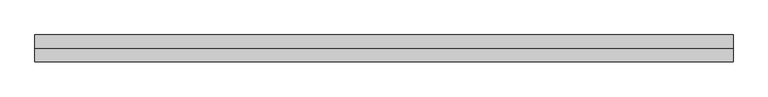
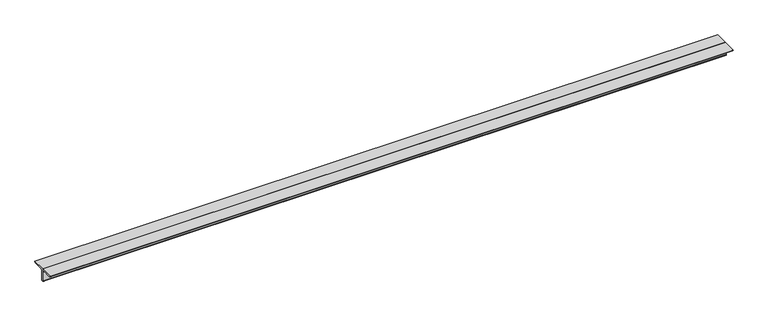
"""IFC4 building model written with IfcOpenShell, lengths in millimetres: member geometry, Steel Framing_2Ls_KS : H_SB_AR_S02_2Ls-100x100x10_VBR1."""

import ifcopenshell
import ifcopenshell.guid

model = None  # the IFC model being written
_history = None  # IfcOwnerHistory: only IFC2X3 demands one
_inside = {}  # id of a spatial element -> (the spatial element, [elements in it])
_under = {}  # id of a project, library or spatial element -> (it, [spatial elements below it])
_declared = {}  # id of a project -> (the project, [libraries it declares])
_typed = {}  # id of a type object -> (the type object, [elements of that type])
_made_of = {}  # id of a material, layer set ... -> (it, [elements and type objects made of it])


def new_model(schema):
    """Start an empty IFC model of exactly this schema.

    Asked for "IFC4X3", IfcOpenShell would pick the latest addendum, in which some entities
    have other attributes; the version numbers below select the first issue.
    IFC2X3 requires an IfcOwnerHistory on every rooted entity: one is made here for all.
    """
    global model, _history
    if schema == "IFC4X3":
        model = ifcopenshell.file(schema_version=(4, 3, 0, 0))
    else:
        model = ifcopenshell.file(schema=schema)
    _inside.clear()
    _under.clear()
    _declared.clear()
    _typed.clear()
    _made_of.clear()
    _history = None
    if model.schema == "IFC2X3":
        org = make("IfcOrganization", Name="unknown")
        user = make(
            "IfcPersonAndOrganization",
            ThePerson=make("IfcPerson", FamilyName="unknown"),
            TheOrganization=org,
        )
        app = make(
            "IfcApplication",
            ApplicationDeveloper=org,
            Version="unknown",
            ApplicationFullName="unknown",
            ApplicationIdentifier="unknown",
        )
        _history = make(
            "IfcOwnerHistory",
            OwningUser=user,
            OwningApplication=app,
            ChangeAction="ADDED",
            CreationDate=0,
        )
    return model


def make(cls, **values):
    """One entity of the class cls with the attributes given. An attribute that is None is left unset."""
    return model.create_entity(
        cls, **{name: value for name, value in values.items() if value is not None}
    )


def rooted(cls, **values):
    """An entity with a GlobalId (a new one), such as an element, a storey or a relation."""
    return make(cls, GlobalId=ifcopenshell.guid.new(), OwnerHistory=_history, **values)


def si_unit(unit_type, name, prefix=None):
    """IfcSIUnit, for example si_unit("LENGTHUNIT", "METRE", prefix="MILLI")."""
    return make("IfcSIUnit", UnitType=unit_type, Prefix=prefix, Name=name)


def assignment(units):
    """IfcUnitAssignment: the units of a project."""
    return None if units is None else make("IfcUnitAssignment", Units=units)


def point(xyz):
    """IfcCartesianPoint."""
    return None if xyz is None else make("IfcCartesianPoint", Coordinates=xyz)


def direction(xyz):
    """IfcDirection."""
    return None if xyz is None else make("IfcDirection", DirectionRatios=xyz)


def frame(location, z_axis=None, x_axis=None):
    """IfcAxis2Placement3D, a coordinate frame: its origin and axes. An axis left out is left unset."""
    return make(
        "IfcAxis2Placement3D",
        Location=point(location),
        Axis=direction(z_axis),
        RefDirection=direction(x_axis),
    )


def frame_2d(location, x_axis=None):
    """IfcAxis2Placement2D, a coordinate frame in the plane: its origin and x axis."""
    return make(
        "IfcAxis2Placement2D", Location=point(location), RefDirection=direction(x_axis)
    )


def origin():
    """The frame at (0, 0, 0) with its axes left unset."""
    return frame((0.0, 0.0, 0.0))


def place(relative_to, where):
    """IfcLocalPlacement: puts the frame where relative to a parent placement (None: the world)."""
    return make(
        "IfcLocalPlacement", PlacementRelTo=relative_to, RelativePlacement=where
    )


def context(
    kind, dimensions, precision=None, world=None, true_north=None, identifier=None
):
    """IfcGeometricRepresentationContext, for example the 3D "Model" context."""
    return make(
        "IfcGeometricRepresentationContext",
        ContextIdentifier=identifier,
        ContextType=kind,
        CoordinateSpaceDimension=dimensions,
        Precision=precision,
        WorldCoordinateSystem=world,
        TrueNorth=true_north,
    )


def project(units=None, contexts=None):
    """IfcProject with its units and contexts."""
    return rooted(
        "IfcProject",
        Name="project",
        RepresentationContexts=contexts,
        UnitsInContext=assignment(units),
    )


def spatial(cls, under=None, at=None, **own):
    """A site, building, storey or space (cls), placed at a placement, below another one or the project."""
    s = rooted(cls, ObjectPlacement=at, **own)
    if under is not None:
        _under.setdefault(under.id(), (under, []))[1].append(s)
    return s


def polyline(points):
    """IfcPolyline through the points."""
    return make("IfcPolyline", Points=[point(p) for p in points])


def circle_curve(where, radius):
    """IfcCircle in the frame where."""
    return make("IfcCircle", Position=where, Radius=radius)


def trimmed(basis, trim1, trim2, sense, master):
    """IfcTrimmedCurve: the piece of a basis curve between two trims."""
    return make(
        "IfcTrimmedCurve",
        BasisCurve=basis,
        Trim1=trim1,
        Trim2=trim2,
        SenseAgreement=sense,
        MasterRepresentation=master,
    )


def segment(curve, same_sense, transition):
    """IfcCompositeCurveSegment."""
    return make(
        "IfcCompositeCurveSegment",
        Transition=transition,
        SameSense=same_sense,
        ParentCurve=curve,
    )


def composite_curve(segments, self_intersect=None):
    """IfcCompositeCurve: segments joined end to end."""
    return make("IfcCompositeCurve", Segments=segments, SelfIntersect=self_intersect)


def outline(outer, holes=None, kind="AREA"):
    """IfcArbitraryClosedProfileDef: a profile drawn as a closed curve; with holes, ...WithVoids."""
    if holes is None:
        return make("IfcArbitraryClosedProfileDef", ProfileType=kind, OuterCurve=outer)
    return make(
        "IfcArbitraryProfileDefWithVoids",
        ProfileType=kind,
        OuterCurve=outer,
        InnerCurves=holes,
    )


def extrude(swept, where, along, depth):
    """IfcExtrudedAreaSolid: the profile swept, set in the frame where, extruded along a direction by depth."""
    return make(
        "IfcExtrudedAreaSolid",
        SweptArea=swept,
        Position=where,
        ExtrudedDirection=direction(along),
        Depth=depth,
    )


def shape(context_of_items, identifier, shape_type, items):
    """IfcShapeRepresentation: the items that make up one representation, for example the "Body"."""
    return make(
        "IfcShapeRepresentation",
        ContextOfItems=context_of_items,
        RepresentationIdentifier=identifier,
        RepresentationType=shape_type,
        Items=items,
    )


def source(mapping_origin, context_of_items, identifier, shape_type, items):
    """IfcRepresentationMap: a shape defined once, which mapped items show again and again."""
    return make(
        "IfcRepresentationMap",
        MappingOrigin=mapping_origin,
        MappedRepresentation=shape(context_of_items, identifier, shape_type, items),
    )


def transform(
    local_origin,
    x_axis=None,
    y_axis=None,
    z_axis=None,
    scale=None,
    scale2=None,
    scale3=None,
    uniform=True,
):
    """IfcCartesianTransformationOperator3D, or its non-uniform kind. x_axis, y_axis, z_axis: its Axis1, 2, 3."""
    if uniform:
        return make(
            "IfcCartesianTransformationOperator3D",
            Axis1=direction(x_axis),
            Axis2=direction(y_axis),
            LocalOrigin=point(local_origin),
            Scale=scale,
            Axis3=direction(z_axis),
        )
    return make(
        "IfcCartesianTransformationOperator3DnonUniform",
        Axis1=direction(x_axis),
        Axis2=direction(y_axis),
        LocalOrigin=point(local_origin),
        Scale=scale,
        Axis3=direction(z_axis),
        Scale2=scale2,
        Scale3=scale3,
    )


def mapped(mapping_source, mapping_target):
    """IfcMappedItem: shows the shape of a source again, moved by a transform."""
    return make(
        "IfcMappedItem", MappingSource=mapping_source, MappingTarget=mapping_target
    )


def made_of(thing, what):
    """Note that an element or type object is made of a material, layer set ...; save() writes the relation."""
    if what is not None:
        _made_of.setdefault(what.id(), (what, []))[1].append(thing)
    return thing


def element(
    cls,
    number,
    at=None,
    inside=None,
    cuts=None,
    type_object=None,
    material=None,
    context=None,
    identifier="Body",
    shape_type=None,
    held_by="IfcProductDefinitionShape",
    body=None,
    shapes=None,
    **own,
):
    """One element of the class cls, such as IfcWall. Its Tag is "e" and its number.

    at: its placement. inside: the storey or other place that contains it. cuts: it is an
    opening in that element (IfcRelVoidsElement). A single representation is given by context,
    identifier, shape_type and body (its items); several are given by shapes. held_by: the class
    of the entity that holds the representations. save() writes the other relations.
    """
    e = rooted(cls, Tag="e%d" % number, ObjectPlacement=at, **own)
    if body is not None:
        shapes = [shape(context, identifier, shape_type, body)]
    if shapes is not None:
        e.Representation = make(held_by, Representations=shapes)
    if inside is not None:
        _inside.setdefault(inside.id(), (inside, []))[1].append(e)
    if cuts is not None:
        rooted(
            "IfcRelVoidsElement", RelatingBuildingElement=cuts, RelatedOpeningElement=e
        )
    if type_object is not None:
        _typed.setdefault(type_object.id(), (type_object, []))[1].append(e)
    return made_of(e, material)


def aggregate(whole, parts):
    """IfcRelAggregates: a whole, such as a stair, and the parts it consists of."""
    return rooted("IfcRelAggregates", RelatingObject=whole, RelatedObjects=parts)


def save(model, path):
    """Write the relations noted so far, then the file.

    IfcRelAggregates (storeys below a building ...), IfcRelContainedInSpatialStructure (elements
    in a storey), IfcRelDefinesByType, IfcRelAssociatesMaterial and IfcRelDeclares: one each for
    every whole, place, type object, material and project.
    """
    for whole, parts in _under.values():
        aggregate(whole, parts)
    for where, things in _inside.values():
        rooted(
            "IfcRelContainedInSpatialStructure",
            RelatedElements=things,
            RelatingStructure=where,
        )
    for kind, things in _typed.values():
        rooted("IfcRelDefinesByType", RelatedObjects=things, RelatingType=kind)
    for what, things in _made_of.values():
        rooted("IfcRelAssociatesMaterial", RelatedObjects=things, RelatingMaterial=what)
    for by, libraries in _declared.values():
        rooted("IfcRelDeclares", RelatingContext=by, RelatedDefinitions=libraries)
    model.write(path)


def member_7627e254(model_context):
    return source(origin(), model_context, "Body", "SweptSolid", [
        extrude(outline(composite_curve([segment(polyline([(0.0, 28.2), (100.0, 28.2)]), True, "CONTINUOUS"), segment(trimmed(circle_curve(frame_2d((90.0, 28.2)), 10.0), [point((100.0, 28.2))], [point((90.0, 18.2))], False, "CARTESIAN"), True, "CONTINUOUS"), segment(polyline([(90.0, 18.2), (20.0, 18.2)]), True, "CONTINUOUS"), segment(trimmed(circle_curve(frame_2d((20.0, 8.2)), 10.0), [point((20.0, 18.2))], [point((10.0, 8.2))], True, "CARTESIAN"), True, "CONTINUOUS"), segment(polyline([(10.0, 8.2), (10.0, -61.8)]), True, "CONTINUOUS"), segment(trimmed(circle_curve(frame_2d((0.0, -61.8)), 10.0), [point((10.0, -61.8))], [point((0.0, -71.8))], False, "CARTESIAN"), True, "CONTINUOUS"), segment(polyline([(0.0, -71.8), (0.0, 28.2)]), True, "CONTINUOUS")], self_intersect=False)), frame((-2590.3354834, 0.0, 0.0), z_axis=(1.0, 0.0, 0.0), x_axis=(0.0, 1.0, 0.0)), (0.0, 0.0, 1.0), 5180.6709668),
        extrude(outline(composite_curve([segment(polyline([(0.0, 28.2), (0.0, -71.8)]), True, "CONTINUOUS"), segment(trimmed(circle_curve(frame_2d((0.0, -61.8)), 10.0), [point((0.0, -71.8))], [point((-10.0, -61.8))], False, "CARTESIAN"), True, "CONTINUOUS"), segment(polyline([(-10.0, -61.8), (-10.0, 8.2)]), True, "CONTINUOUS"), segment(trimmed(circle_curve(frame_2d((-20.0, 8.2)), 10.0), [point((-10.0, 8.2))], [point((-20.0, 18.2))], True, "CARTESIAN"), True, "CONTINUOUS"), segment(polyline([(-20.0, 18.2), (-90.0, 18.2)]), True, "CONTINUOUS"), segment(trimmed(circle_curve(frame_2d((-90.0, 28.2)), 10.0), [point((-90.0, 18.2))], [point((-100.0, 28.2))], False, "CARTESIAN"), True, "CONTINUOUS"), segment(polyline([(-100.0, 28.2), (0.0, 28.2)]), True, "CONTINUOUS")], self_intersect=False)), frame((-2590.3354834, 0.0, 0.0), z_axis=(1.0, 0.0, 0.0), x_axis=(0.0, 1.0, 0.0)), (0.0, 0.0, 1.0), 5180.6709668),
    ])


if __name__ == "__main__":
    model = new_model("IFC4")
    model_context = context("Model", 3, world=origin())
    ifc_project = project(units=[si_unit("LENGTHUNIT", "METRE", prefix="MILLI")], contexts=[model_context])
    site = spatial("IfcSite", under=ifc_project)
    building = spatial("IfcBuilding", under=site)
    placement = place(None, origin())
    member_shape = member_7627e254(model_context)
    element("IfcMember", 1, ObjectType="Steel Framing_2Ls_KS : H_SB_AR_S02_2Ls-100x100x10_VBR1", at=placement, inside=building, context=model_context, shape_type="MappedRepresentation", body=[
        mapped(member_shape, transform((0.0, 0.0, 0.0), x_axis=(1.0, 0.0, 0.0), y_axis=(0.0, 1.0, 0.0), z_axis=(0.0, 0.0, 1.0))),
    ])
    save(model, "model.ifc")

# Revit data of these elements
# Type "Steel Framing_2Ls_KS : H_SB_AR_S02_2Ls-100x100x10_VBR1"
#   Type Comments = "MAIN"
#   Type Mark = "VBR1"
#   H_SectionID = "2Ls-100x100x10"
#   Assembly Code = "B10"
#   Legs = "LLBB"
#   H_Ratio for Additional Steel Plate = 0.2
#   W = 0
#   Perimeter = 0.80 m²/m
#   Nominal Weight = 29.80 kgf/m
#   Length [instance default] = 1524 mm
#   Space = 0 mm
#   b = 100 mm
#   d = 100 mm
#   t = 10 mm
#   y = 28.2 mm
#   A = 0.0038 m²
#   Structural Material [instance default] = Steel, 45-345
# Element 1 (IfcMember, "Steel Framing_2Ls_KS : H_SB_AR_S02_2Ls-100x100x10_VBR1")
#   Materials on its faces: "Steel, 45-345"
# Materials
#   "Steel, 45-345": class "Metal", colour RGB 189 187 185, transparency 0, Description = "Steel 345 MPa", Cost = 0
